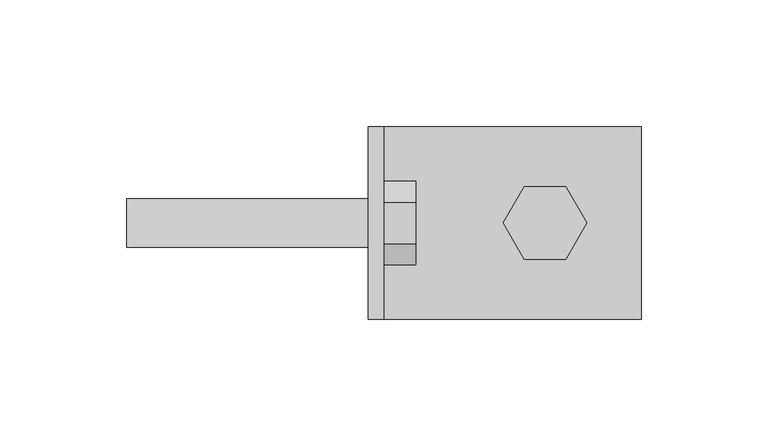
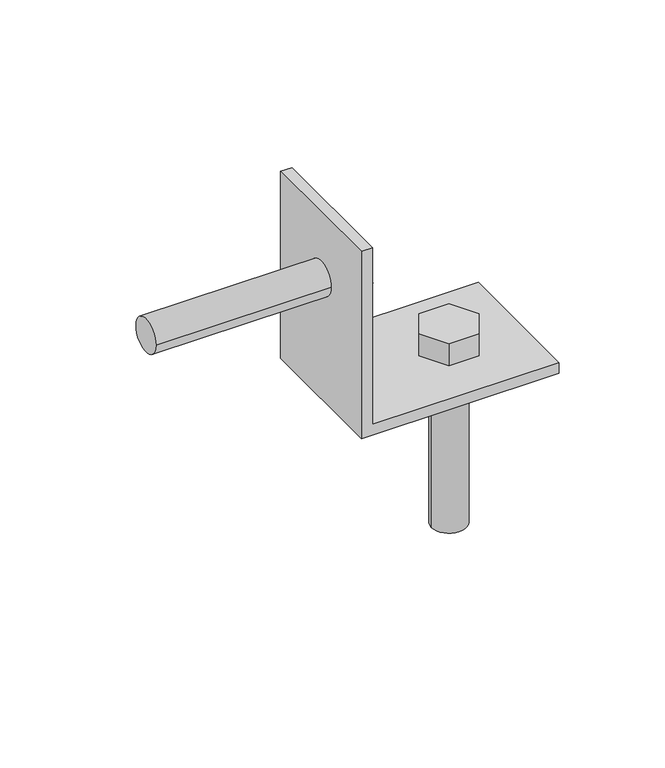
"""IFC4 building model written with IfcOpenShell, lengths in millimetres: fastener geometry, SIMPSON - HLPC/HLGPC Heavy Angles and Gussets : SIMPSON - HL43 - 3 X 4.25 - .75 Bolt - HDG."""

from ifc_helpers import new_model, si_unit, point, frame, frame_2d, origin, place, context, project, spatial, polyline, circle_curve, trimmed, segment, composite_curve, outline, extrude, source, transform, mapped, element, save
from ifc_brep_helpers import plane_surface, revolved_surface, advanced_brep


def fastener_c5b4ea8f(model_context):
    return source(origin(), model_context, "Body", "SolidModel", [
        extrude(outline(composite_curve([segment(trimmed(circle_curve(frame_2d((0.0, 69.85)), 9.525), [point((-9.525, 69.85))], [point((9.525, 69.85))], False, "CARTESIAN"), True, "CONTINUOUS"), segment(trimmed(circle_curve(frame_2d((0.0, 69.85)), 9.525), [point((9.525, 69.85))], [point((-9.525, 69.85))], False, "CARTESIAN"), True, "CONTINUOUS")], self_intersect=False)), frame((-95.5476562, 0.0, 0.0), z_axis=(1.0, 0.0, 0.0), x_axis=(0.0, 1.0, 0.0)), (0.0, 0.0, 1.0), 101.6),
        extrude(outline(polyline([(-16.4977839, 69.85), (-8.248892, 84.1375), (8.248892, 84.1375), (16.4977839, 69.85), (8.248892, 55.5625), (-8.248892, 55.5625), (-16.4977839, 69.85)])), frame((6.0523438, 0.0, 0.0), z_axis=(1.0, 0.0, 0.0), x_axis=(0.0, 1.0, 0.0)), (0.0, 0.0, 1.0), 12.7),
        extrude(outline(composite_curve([segment(trimmed(circle_curve(frame_2d((69.85, 0.0)), 9.525), [point((60.325, 0.0))], [point((79.375, 0.0))], False, "CARTESIAN"), True, "CONTINUOUS"), segment(trimmed(circle_curve(frame_2d((69.85, 0.0)), 9.525), [point((79.375, 0.0))], [point((60.325, 0.0))], False, "CARTESIAN"), True, "CONTINUOUS")], self_intersect=False)), frame((0.0, 0.0, -95.5476563), z_axis=(0.0, 0.0, 1.0), x_axis=(1.0, 0.0, 0.0)), (0.0, 0.0, 1.0), 101.6),
        extrude(outline(polyline([(53.3522161, 0.0), (61.601108, 14.2875), (78.098892, 14.2875), (86.3477839, 0.0), (78.098892, -14.2875), (61.601108, -14.2875), (53.3522161, 0.0)])), frame((0.0, 0.0, 6.0523437), z_axis=(0.0, 0.0, 1.0), x_axis=(1.0, 0.0, 0.0)), (0.0, 0.0, 1.0), 12.7),
        advanced_brep(
        [(6.0523438, 38.1, 107.95), (6.0523438, -38.1, 107.95), (6.0523438, -38.1, 6.0523437), (6.0523438, 38.1, 6.0523437), (6.0523438, 9.525, 69.85), (6.0523438, -9.525, 69.85), (0.0, -38.1, 107.95), (0.0, 38.1, 107.95), (0.0, 38.1, 0.0), (0.0, -38.1, 0.0), (0.0, -9.525, 69.85), (0.0, 9.525, 69.85), (107.95, -38.1, 0.0), (107.95, -38.1, 6.0523437), (107.95, 38.1, 6.0523437), (107.95, 38.1, 0.0), (79.375, 0.0, 6.0523437), (60.325, 0.0, 6.0523437), (60.325, 0.0, 0.0), (79.375, 0.0, 0.0)],
        [
            (0, 1),
            (1, 2),
            (2, 3),
            (3, 0),
            (4, 5, circle_curve(frame((6.0523438, 0.0, 69.85), z_axis=(-1.0, 0.0, 0.0), x_axis=(0.0, 1.0, 0.0)), 9.525)),
            (5, 4, circle_curve(frame((6.0523438, 0.0, 69.85), z_axis=(-1.0, 0.0, 0.0), x_axis=(0.0, 1.0, 0.0)), 9.525)),
            (6, 7),
            (7, 8),
            (8, 9),
            (9, 6),
            (10, 11, circle_curve(frame((0.0, 0.0, 69.85), z_axis=(1.0, 0.0, 0.0), x_axis=(0.0, 1.0, 0.0)), 9.525)),
            (11, 10, circle_curve(frame((0.0, 0.0, 69.85), z_axis=(1.0, 0.0, 0.0), x_axis=(0.0, 1.0, 0.0)), 9.525)),
            (0, 7),
            (6, 1),
            (9, 12),
            (12, 13),
            (13, 2),
            (3, 14),
            (14, 15),
            (15, 8),
            (13, 14),
            (16, 17, circle_curve(frame((69.85, 0.0, 6.0523437), z_axis=(0.0, 0.0, -1.0), x_axis=(1.0, 0.0, 0.0)), 9.525)),
            (17, 16, circle_curve(frame((69.85, 0.0, 6.0523437), z_axis=(0.0, 0.0, -1.0), x_axis=(1.0, 0.0, 0.0)), 9.525)),
            (15, 12),
            (18, 19, circle_curve(frame((69.85, 0.0, 0.0), z_axis=(0.0, 0.0, 1.0), x_axis=(1.0, 0.0, 0.0)), 9.525)),
            (19, 18, circle_curve(frame((69.85, 0.0, 0.0), z_axis=(0.0, 0.0, 1.0), x_axis=(1.0, 0.0, 0.0)), 9.525)),
            (16, 19),
            (18, 17),
            (4, 11),
            (10, 5),
        ],
        [
            plane_surface(frame((6.0523438, -38.1, 107.95), z_axis=(1.0, 0.0, 0.0), x_axis=(0.0, -1.0, 0.0))),
            plane_surface(frame((0.0, -38.1, 107.95), z_axis=(-1.0, 0.0, 0.0), x_axis=(0.0, 1.0, 0.0))),
            plane_surface(frame((6.0523438, 38.1, 107.95), z_axis=(0.0, 0.0, 1.0), x_axis=(-1.0, 0.0, 0.0))),
            plane_surface(frame((6.0523438, -38.1, 107.95), z_axis=(0.0, -1.0, 0.0), x_axis=(-1.0, 0.0, 0.0))),
            plane_surface(frame((6.0523438, 38.1, 6.0523437), z_axis=(0.0, 1.0, 0.0), x_axis=(-1.0, 0.0, 0.0))),
            plane_surface(frame((0.0, 38.1, 6.0523437), z_axis=(0.0, 0.0, 1.0), x_axis=(-1.0, 0.0, 0.0))),
            plane_surface(frame((0.0, 38.1, 0.0), z_axis=(0.0, 0.0, -1.0), x_axis=(1.0, 0.0, 0.0))),
            plane_surface(frame((107.95, -38.1, 6.0523437), z_axis=(1.0, 0.0, 0.0), x_axis=(0.0, 0.0, -1.0))),
            revolved_surface(polyline([(79.375, 0.0, 6.0523437), (79.375, 0.0, 0.0)]), (69.85, 0.0, 0.0), (0.0, 0.0, 1.0)),
            revolved_surface(polyline([(6.0523438, 9.525, 69.85), (0.0, 9.525, 69.85)]), (0.0, 0.0, 69.85), (1.0, 0.0, 0.0)),
        ],
        [
            (0, [[1, 2, 3, 4], [5, 6]]),
            (1, [[7, 8, 9, 10], [11, 12]]),
            (2, [[-1, 13, -7, 14]]),
            (3, [[-2, -14, -10, 15, 16, 17]]),
            (4, [[-4, 18, 19, 20, -8, -13]]),
            (5, [[21, -18, -3, -17], [22, 23]]),
            (6, [[24, -15, -9, -20], [25, 26]]),
            (7, [[-21, -16, -24, -19]]),
            (8, [[27, -25, 28, -22]]),
            (8, [[-27, -23, -28, -26]]),
            (9, [[29, -11, 30, -5]]),
            (9, [[-29, -6, -30, -12]]),
        ],
    ),
    ])


if __name__ == "__main__":
    model = new_model("IFC4")
    model_context = context("Model", 3, world=origin())
    ifc_project = project(units=[si_unit("LENGTHUNIT", "METRE", prefix="MILLI")], contexts=[model_context])
    site = spatial("IfcSite", under=ifc_project)
    building = spatial("IfcBuilding", under=site)
    placement = place(None, origin())
    fastener_shape = fastener_c5b4ea8f(model_context)
    element("IfcFastener", 1, ObjectType="SIMPSON - HLPC/HLGPC Heavy Angles and Gussets : SIMPSON - HL43 - 3 X 4.25 - .75 Bolt - HDG", at=placement, inside=building, context=model_context, shape_type="MappedRepresentation", body=[
        mapped(fastener_shape, transform((0.0, 0.0, 0.0), x_axis=(1.0, 0.0, 0.0), y_axis=(0.0, 1.0, 0.0), z_axis=(0.0, 0.0, 1.0))),
    ])
    save(model, "model.ifc")

# Revit data of these elements
# Type "SIMPSON - HLPC/HLGPC Heavy Angles and Gussets : SIMPSON - HL43 - 3 X 4.25 - .75 Bolt - HDG"
#   URL = "https://www.strongtie.com/classiccollection_architecturalproductsgroup/hlpc-hlgpc_productgroup_wcc/p/hlpc.hlgpc"
#   L = 0' - 3"
#   Hole Radius = 0' - 0 3/8"
#   D4 = 0' - 5"
#   D2 = 0' - 5"
#   D1 = 0' - 1 1/2"
#   D3 = 0' - 2 3/4"
#   Ga. = 0' - 0 61/256"
#   W1 & W2 = 0' - 4 1/4"
#   Default Elevation = 4' - 0"
#   Bolt Visibility - 3B = no
#   Bolt Visibility - 3A = no
#   Bolt Visibility - 2B = no
#   Bolt Visibility - 2A = no
#   Bolt Visibility - 1B = no
#   Bolt Visibility - 1A = yes
#   Bolt Visibility = yes
#   Bolt Size = element 1298415
# Element 1 (IfcFastener, "SIMPSON - HLPC/HLGPC Heavy Angles and Gussets : SIMPSON - HL43 - 3 X 4.25 - .75 Bolt - HDG")
#   Materials on its faces: "1\" GALV. LAG BOLT (LENGTH = 1/2\" SHY OF GLULAM DEPTH) -  (GALV. THRU BOLT IF PLATE ON OPP. SIDE OF STRUCT MEMBER)"
# Materials
#   "1\" GALV. LAG BOLT (LENGTH = 1/2\" SHY OF GLULAM DEPTH) -  (GALV. THRU BOLT IF PLATE ON OPP. SIDE OF STRUCT MEMBER)": class "Generic", colour RGB 120 120 120, transparency 0, Cost = 0
